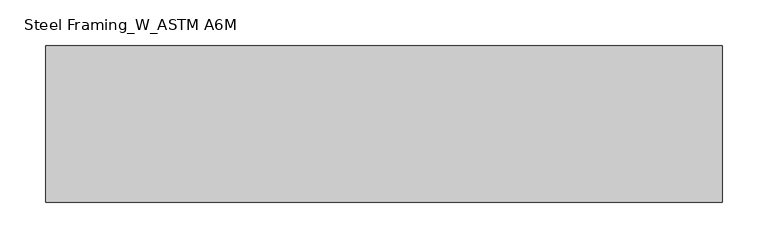
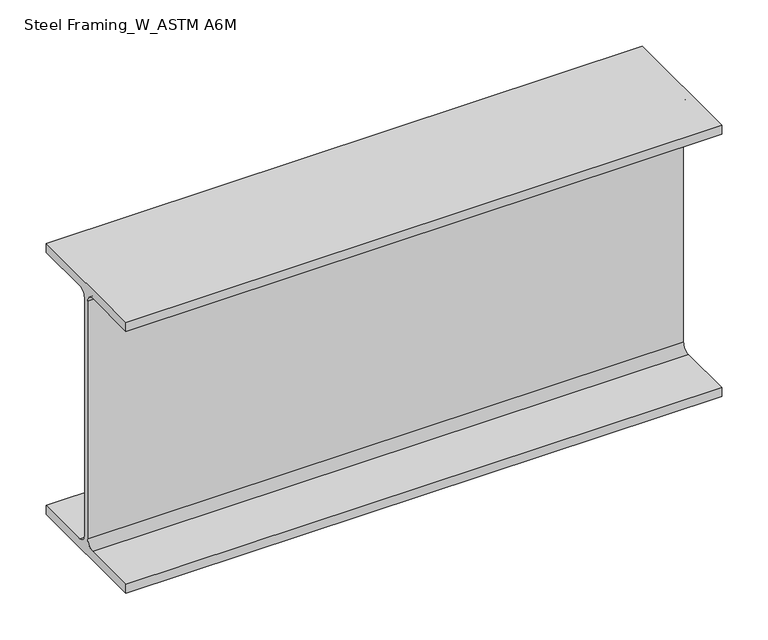
"""IFC4 building model written with IfcOpenShell, lengths in millimetres: beam geometry, Steel Framing_W_ASTM A6M : H_SB_AR_S02_W360x51_RG1."""

import ifcopenshell
import ifcopenshell.guid

model = None  # the IFC model being written
_history = None  # IfcOwnerHistory: only IFC2X3 demands one
_inside = {}  # id of a spatial element -> (the spatial element, [elements in it])
_under = {}  # id of a project, library or spatial element -> (it, [spatial elements below it])
_declared = {}  # id of a project -> (the project, [libraries it declares])
_typed = {}  # id of a type object -> (the type object, [elements of that type])
_made_of = {}  # id of a material, layer set ... -> (it, [elements and type objects made of it])


def new_model(schema):
    """Start an empty IFC model of exactly this schema.

    Asked for "IFC4X3", IfcOpenShell would pick the latest addendum, in which some entities
    have other attributes; the version numbers below select the first issue.
    IFC2X3 requires an IfcOwnerHistory on every rooted entity: one is made here for all.
    """
    global model, _history
    if schema == "IFC4X3":
        model = ifcopenshell.file(schema_version=(4, 3, 0, 0))
    else:
        model = ifcopenshell.file(schema=schema)
    _inside.clear()
    _under.clear()
    _declared.clear()
    _typed.clear()
    _made_of.clear()
    _history = None
    if model.schema == "IFC2X3":
        org = make("IfcOrganization", Name="unknown")
        user = make(
            "IfcPersonAndOrganization",
            ThePerson=make("IfcPerson", FamilyName="unknown"),
            TheOrganization=org,
        )
        app = make(
            "IfcApplication",
            ApplicationDeveloper=org,
            Version="unknown",
            ApplicationFullName="unknown",
            ApplicationIdentifier="unknown",
        )
        _history = make(
            "IfcOwnerHistory",
            OwningUser=user,
            OwningApplication=app,
            ChangeAction="ADDED",
            CreationDate=0,
        )
    return model


def make(cls, **values):
    """One entity of the class cls with the attributes given. An attribute that is None is left unset."""
    return model.create_entity(
        cls, **{name: value for name, value in values.items() if value is not None}
    )


def rooted(cls, **values):
    """An entity with a GlobalId (a new one), such as an element, a storey or a relation."""
    return make(cls, GlobalId=ifcopenshell.guid.new(), OwnerHistory=_history, **values)


def si_unit(unit_type, name, prefix=None):
    """IfcSIUnit, for example si_unit("LENGTHUNIT", "METRE", prefix="MILLI")."""
    return make("IfcSIUnit", UnitType=unit_type, Prefix=prefix, Name=name)


def assignment(units):
    """IfcUnitAssignment: the units of a project."""
    return None if units is None else make("IfcUnitAssignment", Units=units)


def point(xyz):
    """IfcCartesianPoint."""
    return None if xyz is None else make("IfcCartesianPoint", Coordinates=xyz)


def direction(xyz):
    """IfcDirection."""
    return None if xyz is None else make("IfcDirection", DirectionRatios=xyz)


def frame(location, z_axis=None, x_axis=None):
    """IfcAxis2Placement3D, a coordinate frame: its origin and axes. An axis left out is left unset."""
    return make(
        "IfcAxis2Placement3D",
        Location=point(location),
        Axis=direction(z_axis),
        RefDirection=direction(x_axis),
    )


def frame_2d(location, x_axis=None):
    """IfcAxis2Placement2D, a coordinate frame in the plane: its origin and x axis."""
    return make(
        "IfcAxis2Placement2D", Location=point(location), RefDirection=direction(x_axis)
    )


def origin():
    """The frame at (0, 0, 0) with its axes left unset."""
    return frame((0.0, 0.0, 0.0))


def place(relative_to, where):
    """IfcLocalPlacement: puts the frame where relative to a parent placement (None: the world)."""
    return make(
        "IfcLocalPlacement", PlacementRelTo=relative_to, RelativePlacement=where
    )


def context(
    kind, dimensions, precision=None, world=None, true_north=None, identifier=None
):
    """IfcGeometricRepresentationContext, for example the 3D "Model" context."""
    return make(
        "IfcGeometricRepresentationContext",
        ContextIdentifier=identifier,
        ContextType=kind,
        CoordinateSpaceDimension=dimensions,
        Precision=precision,
        WorldCoordinateSystem=world,
        TrueNorth=true_north,
    )


def project(units=None, contexts=None):
    """IfcProject with its units and contexts."""
    return rooted(
        "IfcProject",
        Name="project",
        RepresentationContexts=contexts,
        UnitsInContext=assignment(units),
    )


def spatial(cls, under=None, at=None, **own):
    """A site, building, storey or space (cls), placed at a placement, below another one or the project."""
    s = rooted(cls, ObjectPlacement=at, **own)
    if under is not None:
        _under.setdefault(under.id(), (under, []))[1].append(s)
    return s


def polyline(points):
    """IfcPolyline through the points."""
    return make("IfcPolyline", Points=[point(p) for p in points])


def circle_curve(where, radius):
    """IfcCircle in the frame where."""
    return make("IfcCircle", Position=where, Radius=radius)


def trimmed(basis, trim1, trim2, sense, master):
    """IfcTrimmedCurve: the piece of a basis curve between two trims."""
    return make(
        "IfcTrimmedCurve",
        BasisCurve=basis,
        Trim1=trim1,
        Trim2=trim2,
        SenseAgreement=sense,
        MasterRepresentation=master,
    )


def segment(curve, same_sense, transition):
    """IfcCompositeCurveSegment."""
    return make(
        "IfcCompositeCurveSegment",
        Transition=transition,
        SameSense=same_sense,
        ParentCurve=curve,
    )


def composite_curve(segments, self_intersect=None):
    """IfcCompositeCurve: segments joined end to end."""
    return make("IfcCompositeCurve", Segments=segments, SelfIntersect=self_intersect)


def outline(outer, holes=None, kind="AREA"):
    """IfcArbitraryClosedProfileDef: a profile drawn as a closed curve; with holes, ...WithVoids."""
    if holes is None:
        return make("IfcArbitraryClosedProfileDef", ProfileType=kind, OuterCurve=outer)
    return make(
        "IfcArbitraryProfileDefWithVoids",
        ProfileType=kind,
        OuterCurve=outer,
        InnerCurves=holes,
    )


def extrude(swept, where, along, depth):
    """IfcExtrudedAreaSolid: the profile swept, set in the frame where, extruded along a direction by depth."""
    return make(
        "IfcExtrudedAreaSolid",
        SweptArea=swept,
        Position=where,
        ExtrudedDirection=direction(along),
        Depth=depth,
    )


def shape(context_of_items, identifier, shape_type, items):
    """IfcShapeRepresentation: the items that make up one representation, for example the "Body"."""
    return make(
        "IfcShapeRepresentation",
        ContextOfItems=context_of_items,
        RepresentationIdentifier=identifier,
        RepresentationType=shape_type,
        Items=items,
    )


def source(mapping_origin, context_of_items, identifier, shape_type, items):
    """IfcRepresentationMap: a shape defined once, which mapped items show again and again."""
    return make(
        "IfcRepresentationMap",
        MappingOrigin=mapping_origin,
        MappedRepresentation=shape(context_of_items, identifier, shape_type, items),
    )


def transform(
    local_origin,
    x_axis=None,
    y_axis=None,
    z_axis=None,
    scale=None,
    scale2=None,
    scale3=None,
    uniform=True,
):
    """IfcCartesianTransformationOperator3D, or its non-uniform kind. x_axis, y_axis, z_axis: its Axis1, 2, 3."""
    if uniform:
        return make(
            "IfcCartesianTransformationOperator3D",
            Axis1=direction(x_axis),
            Axis2=direction(y_axis),
            LocalOrigin=point(local_origin),
            Scale=scale,
            Axis3=direction(z_axis),
        )
    return make(
        "IfcCartesianTransformationOperator3DnonUniform",
        Axis1=direction(x_axis),
        Axis2=direction(y_axis),
        LocalOrigin=point(local_origin),
        Scale=scale,
        Axis3=direction(z_axis),
        Scale2=scale2,
        Scale3=scale3,
    )


def mapped(mapping_source, mapping_target):
    """IfcMappedItem: shows the shape of a source again, moved by a transform."""
    return make(
        "IfcMappedItem", MappingSource=mapping_source, MappingTarget=mapping_target
    )


def made_of(thing, what):
    """Note that an element or type object is made of a material, layer set ...; save() writes the relation."""
    if what is not None:
        _made_of.setdefault(what.id(), (what, []))[1].append(thing)
    return thing


def element(
    cls,
    number,
    at=None,
    inside=None,
    cuts=None,
    type_object=None,
    material=None,
    context=None,
    identifier="Body",
    shape_type=None,
    held_by="IfcProductDefinitionShape",
    body=None,
    shapes=None,
    **own,
):
    """One element of the class cls, such as IfcWall. Its Tag is "e" and its number.

    at: its placement. inside: the storey or other place that contains it. cuts: it is an
    opening in that element (IfcRelVoidsElement). A single representation is given by context,
    identifier, shape_type and body (its items); several are given by shapes. held_by: the class
    of the entity that holds the representations. save() writes the other relations.
    """
    e = rooted(cls, Tag="e%d" % number, ObjectPlacement=at, **own)
    if body is not None:
        shapes = [shape(context, identifier, shape_type, body)]
    if shapes is not None:
        e.Representation = make(held_by, Representations=shapes)
    if inside is not None:
        _inside.setdefault(inside.id(), (inside, []))[1].append(e)
    if cuts is not None:
        rooted(
            "IfcRelVoidsElement", RelatingBuildingElement=cuts, RelatedOpeningElement=e
        )
    if type_object is not None:
        _typed.setdefault(type_object.id(), (type_object, []))[1].append(e)
    return made_of(e, material)


def aggregate(whole, parts):
    """IfcRelAggregates: a whole, such as a stair, and the parts it consists of."""
    return rooted("IfcRelAggregates", RelatingObject=whole, RelatedObjects=parts)


def save(model, path):
    """Write the relations noted so far, then the file.

    IfcRelAggregates (storeys below a building ...), IfcRelContainedInSpatialStructure (elements
    in a storey), IfcRelDefinesByType, IfcRelAssociatesMaterial and IfcRelDeclares: one each for
    every whole, place, type object, material and project.
    """
    for whole, parts in _under.values():
        aggregate(whole, parts)
    for where, things in _inside.values():
        rooted(
            "IfcRelContainedInSpatialStructure",
            RelatedElements=things,
            RelatingStructure=where,
        )
    for kind, things in _typed.values():
        rooted("IfcRelDefinesByType", RelatedObjects=things, RelatingType=kind)
    for what, things in _made_of.values():
        rooted("IfcRelAssociatesMaterial", RelatedObjects=things, RelatingMaterial=what)
    for by, libraries in _declared.values():
        rooted("IfcRelDeclares", RelatingContext=by, RelatedDefinitions=libraries)
    model.write(path)


def steel_framing_w_astm_a6m_5bb5b74e(model_context):
    return source(origin(), model_context, "Body", "SweptSolid", [
        extrude(outline(composite_curve([segment(polyline([(85.5, -166.4), (85.5, -178.0), (-85.5, -178.0), (-85.5, -166.4), (-13.72, -166.4)]), True, "CONTINUOUS"), segment(trimmed(circle_curve(frame_2d((-13.72, -156.3)), 10.1), [point((-13.72, -166.4))], [point((-3.62, -156.3))], True, "CARTESIAN"), True, "CONTINUOUS"), segment(polyline([(-3.62, -156.3), (-3.62, 156.3)]), True, "CONTINUOUS"), segment(trimmed(circle_curve(frame_2d((-13.72, 156.3)), 10.1), [point((-3.62, 156.3))], [point((-13.72, 166.4))], True, "CARTESIAN"), True, "CONTINUOUS"), segment(polyline([(-13.72, 166.4), (-85.5, 166.4), (-85.5, 178.0), (85.5, 178.0), (85.5, 166.4), (13.72, 166.4)]), True, "CONTINUOUS"), segment(trimmed(circle_curve(frame_2d((13.72, 156.3)), 10.1), [point((13.72, 166.4))], [point((3.62, 156.3))], True, "CARTESIAN"), True, "CONTINUOUS"), segment(polyline([(3.62, 156.3), (3.62, -156.3)]), True, "CONTINUOUS"), segment(trimmed(circle_curve(frame_2d((13.72, -156.3)), 10.1), [point((3.62, -156.3))], [point((13.72, -166.4))], True, "CARTESIAN"), True, "CONTINUOUS"), segment(polyline([(13.72, -166.4), (85.5, -166.4)]), True, "CONTINUOUS")], self_intersect=False)), frame((-228.4, 0.0, 0.0), z_axis=(1.0, 0.0, 0.0), x_axis=(0.0, 1.0, 0.0)), (0.0, 0.0, 1.0), 739.7),
    ])


if __name__ == "__main__":
    model = new_model("IFC4")
    model_context = context("Model", 3, world=origin())
    ifc_project = project(units=[si_unit("LENGTHUNIT", "METRE", prefix="MILLI")], contexts=[model_context])
    site = spatial("IfcSite", under=ifc_project)
    building = spatial("IfcBuilding", under=site)
    placement = place(None, origin())
    steel_framing_w_astm_a6m_shape = steel_framing_w_astm_a6m_5bb5b74e(model_context)
    element("IfcBeam", 1, ObjectType="Steel Framing_W_ASTM A6M : H_SB_AR_S02_W360x51_RG1", at=placement, inside=building, context=model_context, shape_type="MappedRepresentation", body=[
        mapped(steel_framing_w_astm_a6m_shape, transform((0.0, 0.0, 0.0), x_axis=(1.0, 0.0, 0.0), y_axis=(0.0, 1.0, 0.0), z_axis=(0.0, 0.0, 1.0))),
    ])
    save(model, "model.ifc")

# Revit data of these elements
# Type "Steel Framing_W_ASTM A6M : H_SB_AR_S02_W360x51_RG1"
#   Type Mark = "RG1"
#   Section Name Key = "W14x34"
#   Width = 17.1 cm
#   Web Thickness = 0.724 cm
#   Web Fillet = 1.01 cm
#   Warping Constant = 287000.0 cm⁶
#   Torsional Moment of Inertia = 23.70 cm⁴
#   Section Area = 64.5 cm²
#   Plastic Modulus weak axis = 174.0 cm³
#   Plastic Modulus strong axis = 895.0 cm³
#   Perimeter = 1.36 m²/m
#   Nominal Weight = 51.00 kgf/m
#   Moment of Inertia weak axis = 970.00 cm⁴
#   Moment of Inertia strong axis = 14200.00 cm⁴
#   Height = 35.6 cm
#   Flange Thickness = 1.16 cm
#   Elastic Modulus weak axis = 113.0 cm³
#   Elastic Modulus strong axis = 796.0 cm³
#   Centroid Vertical = 17.8 cm
#   Centroid Horizontal = 8.55 cm
#   Length [instance default] = 1500 mm
#   Structural Material [instance default] = Steel, 45-345
#   Bolt Spacing = 0
#   Assembly Code = ""
# Element 1 (IfcBeam, "Steel Framing_W_ASTM A6M : H_SB_AR_S02_W360x51_RG1")
#   Materials on its faces: "Steel, 45-345"
# Materials
#   "Steel, 45-345": class "Metal", colour RGB 189 187 185, transparency 0, Description = "Steel 345 MPa", Cost = 0
